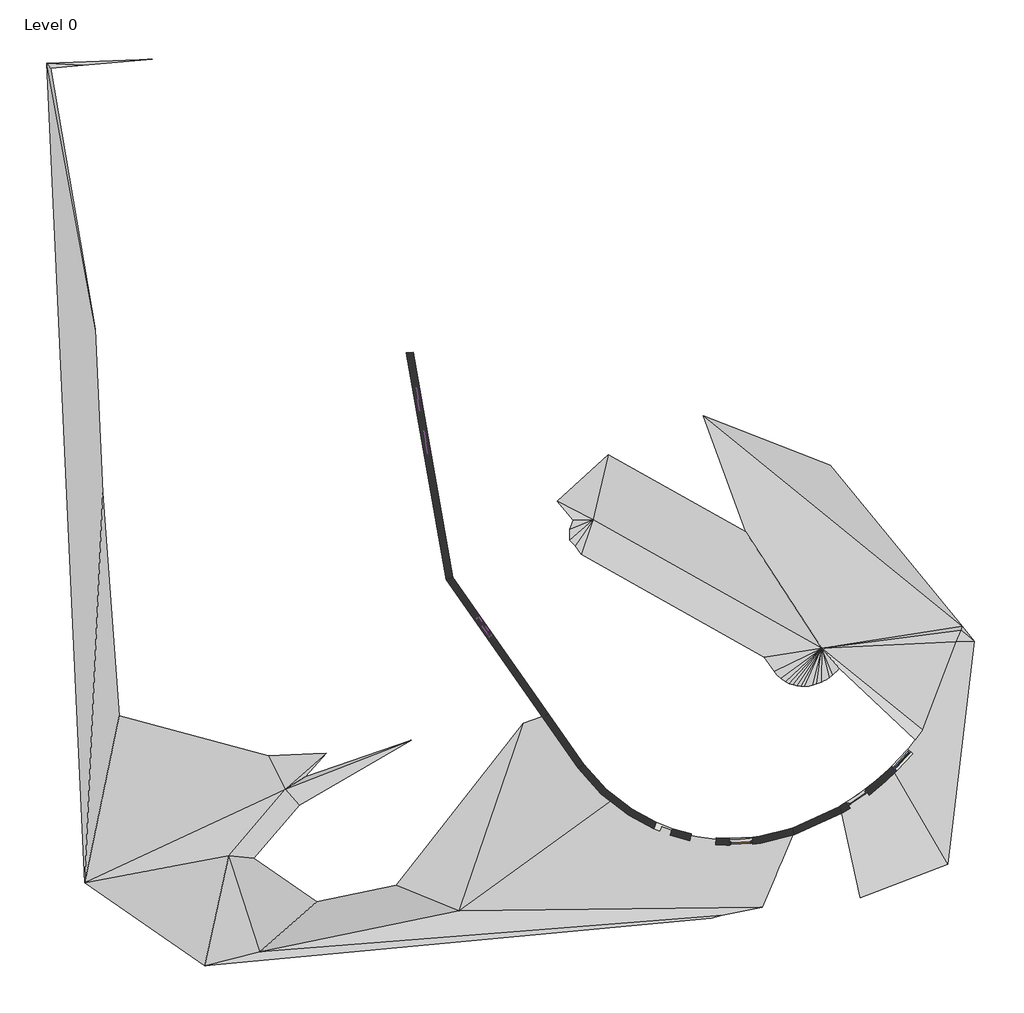
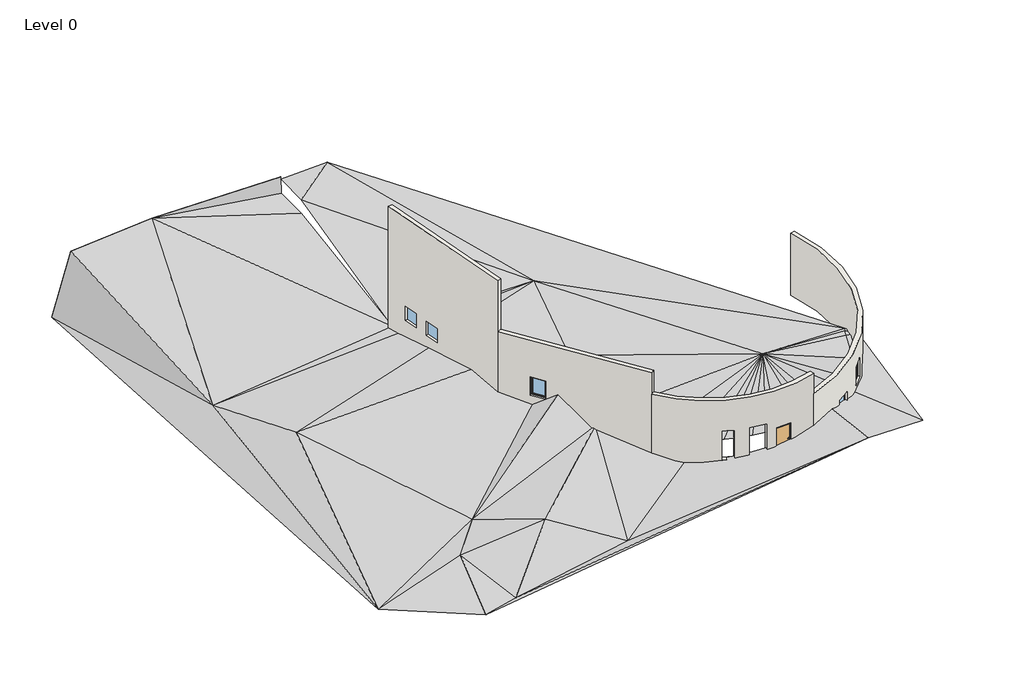
# One storey: 5 windows, 4 walls, 2 proxies, 1 door.
# Revit data of these elements (continued)
# Element 12 (IfcWindow, "Single Window : 10x13 Inåtgående") (continued)
#   Mark = "44"
#   Width = 1010 mm
#   Inset1000 = 1070 mm
#   Inset = 70 mm
#   Height = 1310 mm
#   GapTop = 15 mm
#   GapSecondary = 15 mm
#   GapPrimary = 15 mm
#   GapBottom = 15 mm
#   MWidth = 10
#   MHeight = 13
#   Gap Top = yes
#   Gap Secondary Side = yes
#   Gap Primary Side = yes
#   Gap Bottom = yes
#   Phase Created = New Construction
#   Materials on its faces: "Partier - Generell", "Glas - Generellt", "Default Window Interior"
# Materials
#   "Kartong": class "Generic", colour RGB 240 240 240, transparency 0, Cost = 0
#   "Plexiglas": class "Generic", colour RGB 201 224 223, transparency 0.85, Cost = 0
#   "Default Window Interior": class "Paint", colour RGB 255 255 255, transparency 0, URL = "www.cad-q.se", Description = "Målning", Cost = 0
#   "Default Hardware": class "Generic", colour RGB 127 127 127, transparency 0, Description = "Default Ironmomgery", Cost = 0
#   "Door - Frame/Mullion": class "Wood", colour RGB 212 179 113, transparency 0, Keynote = "L20", Cost = 0
#   "Partier - Generell": class "Generic", colour RGB 153 153 153, transparency 0, URL = "www.cad-q.se", Description = "Odefinierat material", Cost = 0
#   "Glas - Generellt": class "Generic", colour RGB 159 197 217, transparency 0.9, URL = "www.cad-q.se", Description = "Odefinerat Glas", Cost = 0
